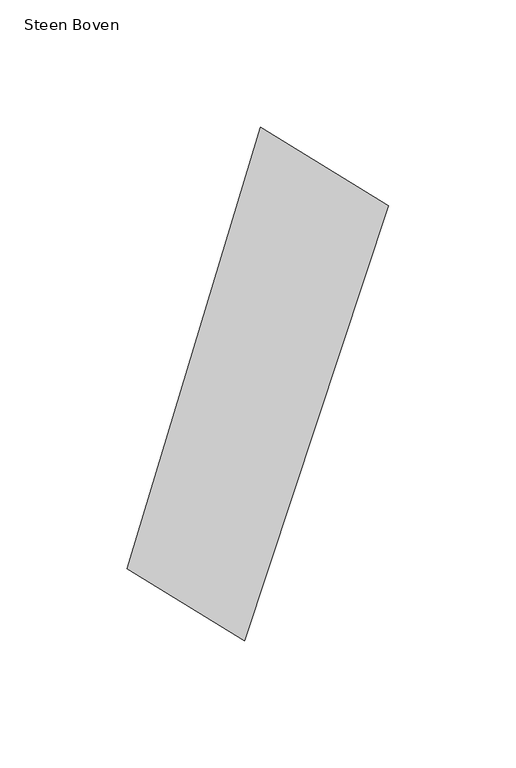
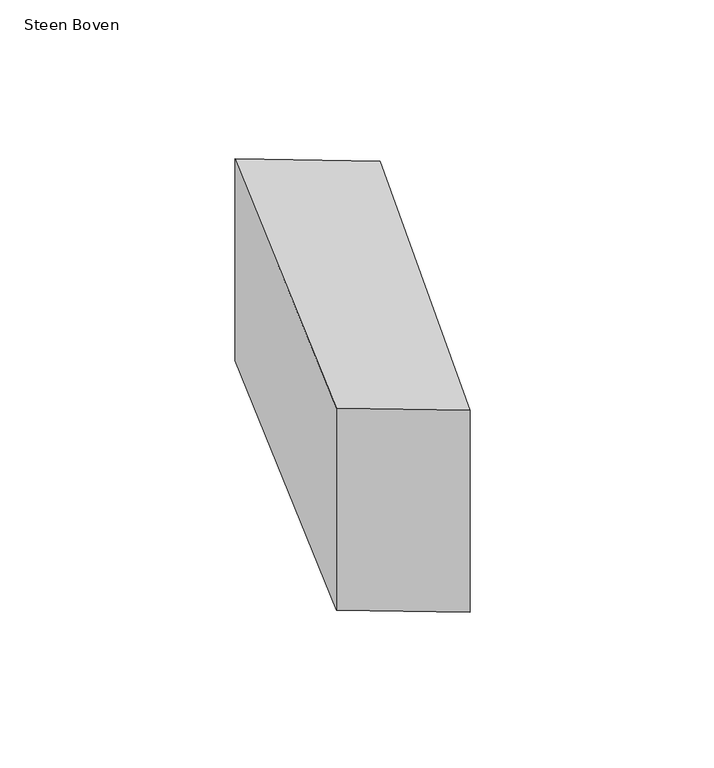
"""IFC4 building model written with IfcOpenShell, lengths in millimetres: proxy geometry, 00_GMA_steen_versie_4 : Steen Boven."""

from ifc_helpers import new_model, si_unit, origin, origin_with_axes, place, context, project, spatial, polyline, outline, extrude, source, transform, mapped, element, save


def steen_boven_1b6bc67c(model_context):
    return source(origin(), model_context, "Body", "SweptSolid", [
        extrude(outline(polyline([(130.3170374, 158.9740552), (73.8313484, -11.8118402), (27.6661823, 16.4443358), (80.0392662, 189.7811639), (130.3170374, 158.9740552)])), origin_with_axes(), (0.0, 0.0, 1.0), 100.0),
    ])


if __name__ == "__main__":
    model = new_model("IFC4")
    model_context = context("Model", 3, world=origin())
    ifc_project = project(units=[si_unit("LENGTHUNIT", "METRE", prefix="MILLI")], contexts=[model_context])
    site = spatial("IfcSite", under=ifc_project)
    building = spatial("IfcBuilding", under=site)
    placement = place(None, origin())
    steen_boven_shape = steen_boven_1b6bc67c(model_context)
    element("IfcBuildingElementProxy", 1, Name="00_GMA_steen_versie_4 : Steen Boven", ObjectType="00_GMA_steen_versie_4 : Steen Boven", at=placement, inside=building, context=model_context, shape_type="MappedRepresentation", body=[
        mapped(steen_boven_shape, transform((0.0, 0.0, 0.0), x_axis=(1.0, 0.0, 0.0), y_axis=(0.0, 1.0, 0.0), z_axis=(0.0, 0.0, 1.0))),
    ])
    save(model, "model.ifc")

# Revit data of these elements
# Type "00_GMA_steen_versie_4 : Steen Boven"
#   StootVoegHalfBoven [instance default] = 5 mm
#   StootVoegHalf [instance default] = 5 mm
#   StootVoegBreedteOnder = 10 mm
#   StootVoegBreedteBoven = 10 mm
#   Steendikte = 100 mm
#   LintVoegOnderHalf = 5 mm
#   LintVoegOnder = 10 mm
#   LintVoegBovenHalf = 0 mm
#   LintVoegBoven = 0 mm
#   materiaal = none
#   MateriaalVoeg = none
#   Default Elevation = 0
